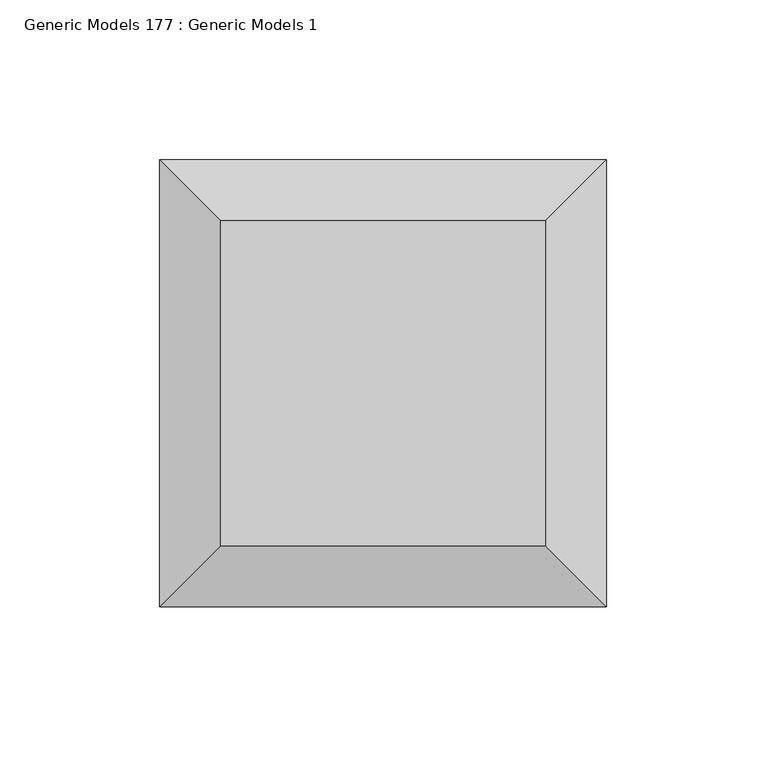
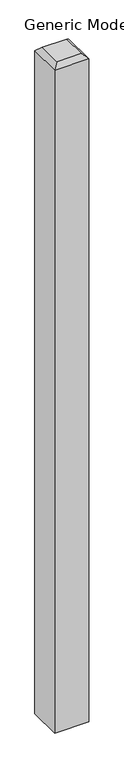
"""IFC4 building model written with IfcOpenShell, lengths in millimetres: proxy geometry, Generic Models 177 : Generic Models 1."""

import ifcopenshell
import ifcopenshell.guid

model = None  # the IFC model being written
_history = None  # IfcOwnerHistory: only IFC2X3 demands one
_inside = {}  # id of a spatial element -> (the spatial element, [elements in it])
_under = {}  # id of a project, library or spatial element -> (it, [spatial elements below it])
_declared = {}  # id of a project -> (the project, [libraries it declares])
_typed = {}  # id of a type object -> (the type object, [elements of that type])
_made_of = {}  # id of a material, layer set ... -> (it, [elements and type objects made of it])


def new_model(schema):
    """Start an empty IFC model of exactly this schema.

    Asked for "IFC4X3", IfcOpenShell would pick the latest addendum, in which some entities
    have other attributes; the version numbers below select the first issue.
    IFC2X3 requires an IfcOwnerHistory on every rooted entity: one is made here for all.
    """
    global model, _history
    if schema == "IFC4X3":
        model = ifcopenshell.file(schema_version=(4, 3, 0, 0))
    else:
        model = ifcopenshell.file(schema=schema)
    _inside.clear()
    _under.clear()
    _declared.clear()
    _typed.clear()
    _made_of.clear()
    _history = None
    if model.schema == "IFC2X3":
        org = make("IfcOrganization", Name="unknown")
        user = make(
            "IfcPersonAndOrganization",
            ThePerson=make("IfcPerson", FamilyName="unknown"),
            TheOrganization=org,
        )
        app = make(
            "IfcApplication",
            ApplicationDeveloper=org,
            Version="unknown",
            ApplicationFullName="unknown",
            ApplicationIdentifier="unknown",
        )
        _history = make(
            "IfcOwnerHistory",
            OwningUser=user,
            OwningApplication=app,
            ChangeAction="ADDED",
            CreationDate=0,
        )
    return model


def make(cls, **values):
    """One entity of the class cls with the attributes given. An attribute that is None is left unset."""
    return model.create_entity(
        cls, **{name: value for name, value in values.items() if value is not None}
    )


def rooted(cls, **values):
    """An entity with a GlobalId (a new one), such as an element, a storey or a relation."""
    return make(cls, GlobalId=ifcopenshell.guid.new(), OwnerHistory=_history, **values)


def si_unit(unit_type, name, prefix=None):
    """IfcSIUnit, for example si_unit("LENGTHUNIT", "METRE", prefix="MILLI")."""
    return make("IfcSIUnit", UnitType=unit_type, Prefix=prefix, Name=name)


def assignment(units):
    """IfcUnitAssignment: the units of a project."""
    return None if units is None else make("IfcUnitAssignment", Units=units)


def point(xyz):
    """IfcCartesianPoint."""
    return None if xyz is None else make("IfcCartesianPoint", Coordinates=xyz)


def direction(xyz):
    """IfcDirection."""
    return None if xyz is None else make("IfcDirection", DirectionRatios=xyz)


def frame(location, z_axis=None, x_axis=None):
    """IfcAxis2Placement3D, a coordinate frame: its origin and axes. An axis left out is left unset."""
    return make(
        "IfcAxis2Placement3D",
        Location=point(location),
        Axis=direction(z_axis),
        RefDirection=direction(x_axis),
    )


def origin():
    """The frame at (0, 0, 0) with its axes left unset."""
    return frame((0.0, 0.0, 0.0))


def place(relative_to, where):
    """IfcLocalPlacement: puts the frame where relative to a parent placement (None: the world)."""
    return make(
        "IfcLocalPlacement", PlacementRelTo=relative_to, RelativePlacement=where
    )


def context(
    kind, dimensions, precision=None, world=None, true_north=None, identifier=None
):
    """IfcGeometricRepresentationContext, for example the 3D "Model" context."""
    return make(
        "IfcGeometricRepresentationContext",
        ContextIdentifier=identifier,
        ContextType=kind,
        CoordinateSpaceDimension=dimensions,
        Precision=precision,
        WorldCoordinateSystem=world,
        TrueNorth=true_north,
    )


def project(units=None, contexts=None):
    """IfcProject with its units and contexts."""
    return rooted(
        "IfcProject",
        Name="project",
        RepresentationContexts=contexts,
        UnitsInContext=assignment(units),
    )


def spatial(cls, under=None, at=None, **own):
    """A site, building, storey or space (cls), placed at a placement, below another one or the project."""
    s = rooted(cls, ObjectPlacement=at, **own)
    if under is not None:
        _under.setdefault(under.id(), (under, []))[1].append(s)
    return s


def faces_of(points, faces, orient=None, outer=None):
    """IfcFace entities. A face is a list of loops; a loop is a list of indices into points, from 0.

    orient and outer hold one flag for each loop. By default every Orientation is true, the
    first loop of a face is its IfcFaceOuterBound and the others are IfcFaceBound.
    """
    made = []
    for i, loops in enumerate(faces):
        bounds = []
        for j, loop in enumerate(loops):
            is_outer = j == 0 if outer is None else outer[i][j]
            bounds.append(
                make(
                    "IfcFaceOuterBound" if is_outer else "IfcFaceBound",
                    Bound=make("IfcPolyLoop", Polygon=[points[k] for k in loop]),
                    Orientation=True if orient is None else orient[i][j],
                )
            )
        made.append(make("IfcFace", Bounds=bounds))
    return made


def faceted_brep(points, faces, orient=None, outer=None, voids=None):
    """IfcFacetedBrep: a solid bounded by flat faces; with voids (closed shells), ...WithVoids."""
    shared = [point(p) for p in points]
    hull = make("IfcClosedShell", CfsFaces=faces_of(shared, faces, orient, outer))
    if voids is None:
        return make("IfcFacetedBrep", Outer=hull)
    return make(
        "IfcFacetedBrepWithVoids",
        Outer=hull,
        Voids=[
            make(cls, CfsFaces=faces_of(shared, fs, o, b)) for cls, fs, o, b in voids
        ],
    )


def shape(context_of_items, identifier, shape_type, items):
    """IfcShapeRepresentation: the items that make up one representation, for example the "Body"."""
    return make(
        "IfcShapeRepresentation",
        ContextOfItems=context_of_items,
        RepresentationIdentifier=identifier,
        RepresentationType=shape_type,
        Items=items,
    )


def source(mapping_origin, context_of_items, identifier, shape_type, items):
    """IfcRepresentationMap: a shape defined once, which mapped items show again and again."""
    return make(
        "IfcRepresentationMap",
        MappingOrigin=mapping_origin,
        MappedRepresentation=shape(context_of_items, identifier, shape_type, items),
    )


def transform(
    local_origin,
    x_axis=None,
    y_axis=None,
    z_axis=None,
    scale=None,
    scale2=None,
    scale3=None,
    uniform=True,
):
    """IfcCartesianTransformationOperator3D, or its non-uniform kind. x_axis, y_axis, z_axis: its Axis1, 2, 3."""
    if uniform:
        return make(
            "IfcCartesianTransformationOperator3D",
            Axis1=direction(x_axis),
            Axis2=direction(y_axis),
            LocalOrigin=point(local_origin),
            Scale=scale,
            Axis3=direction(z_axis),
        )
    return make(
        "IfcCartesianTransformationOperator3DnonUniform",
        Axis1=direction(x_axis),
        Axis2=direction(y_axis),
        LocalOrigin=point(local_origin),
        Scale=scale,
        Axis3=direction(z_axis),
        Scale2=scale2,
        Scale3=scale3,
    )


def mapped(mapping_source, mapping_target):
    """IfcMappedItem: shows the shape of a source again, moved by a transform."""
    return make(
        "IfcMappedItem", MappingSource=mapping_source, MappingTarget=mapping_target
    )


def made_of(thing, what):
    """Note that an element or type object is made of a material, layer set ...; save() writes the relation."""
    if what is not None:
        _made_of.setdefault(what.id(), (what, []))[1].append(thing)
    return thing


def element(
    cls,
    number,
    at=None,
    inside=None,
    cuts=None,
    type_object=None,
    material=None,
    context=None,
    identifier="Body",
    shape_type=None,
    held_by="IfcProductDefinitionShape",
    body=None,
    shapes=None,
    **own,
):
    """One element of the class cls, such as IfcWall. Its Tag is "e" and its number.

    at: its placement. inside: the storey or other place that contains it. cuts: it is an
    opening in that element (IfcRelVoidsElement). A single representation is given by context,
    identifier, shape_type and body (its items); several are given by shapes. held_by: the class
    of the entity that holds the representations. save() writes the other relations.
    """
    e = rooted(cls, Tag="e%d" % number, ObjectPlacement=at, **own)
    if body is not None:
        shapes = [shape(context, identifier, shape_type, body)]
    if shapes is not None:
        e.Representation = make(held_by, Representations=shapes)
    if inside is not None:
        _inside.setdefault(inside.id(), (inside, []))[1].append(e)
    if cuts is not None:
        rooted(
            "IfcRelVoidsElement", RelatingBuildingElement=cuts, RelatedOpeningElement=e
        )
    if type_object is not None:
        _typed.setdefault(type_object.id(), (type_object, []))[1].append(e)
    return made_of(e, material)


def aggregate(whole, parts):
    """IfcRelAggregates: a whole, such as a stair, and the parts it consists of."""
    return rooted("IfcRelAggregates", RelatingObject=whole, RelatedObjects=parts)


def save(model, path):
    """Write the relations noted so far, then the file.

    IfcRelAggregates (storeys below a building ...), IfcRelContainedInSpatialStructure (elements
    in a storey), IfcRelDefinesByType, IfcRelAssociatesMaterial and IfcRelDeclares: one each for
    every whole, place, type object, material and project.
    """
    for whole, parts in _under.values():
        aggregate(whole, parts)
    for where, things in _inside.values():
        rooted(
            "IfcRelContainedInSpatialStructure",
            RelatedElements=things,
            RelatingStructure=where,
        )
    for kind, things in _typed.values():
        rooted("IfcRelDefinesByType", RelatedObjects=things, RelatingType=kind)
    for what, things in _made_of.values():
        rooted("IfcRelAssociatesMaterial", RelatedObjects=things, RelatingMaterial=what)
    for by, libraries in _declared.values():
        rooted("IfcRelDeclares", RelatingContext=by, RelatedDefinitions=libraries)
    model.write(path)


def generic_models_177_generic_models_1_1d143019(model_context):
    return source(origin(), model_context, "Body", "Brep", [
        faceted_brep([(56665.8125, 528.6375, -1066.8), (56526.1125, 528.6375, -1066.8), (56526.1125, 528.6375, 1809.75), (56665.8125, 528.6375, 1809.75), (56665.8125, 388.9375, -1066.8), (56665.8125, 388.9375, 1809.75), (56526.1125, 388.9375, 1809.75), (56526.1125, 388.9375, -1066.8), (56545.1625, 407.9875, 1828.8), (56646.7625, 407.9875, 1828.8), (56646.7625, 509.5875, 1828.8), (56545.1625, 509.5875, 1828.8)], [[[0, 1, 2, 3]], [[4, 5, 6, 7]], [[1, 0, 4, 7]], [[2, 1, 7, 6]], [[8, 9, 10, 11]], [[0, 3, 5, 4]], [[2, 6, 8, 11]], [[5, 3, 10, 9]], [[6, 5, 9, 8]], [[3, 2, 11, 10]]]),
    ])


if __name__ == "__main__":
    model = new_model("IFC4")
    model_context = context("Model", 3, world=origin())
    ifc_project = project(units=[si_unit("LENGTHUNIT", "METRE", prefix="MILLI")], contexts=[model_context])
    site = spatial("IfcSite", under=ifc_project)
    building = spatial("IfcBuilding", under=site)
    placement = place(None, origin())
    generic_models_177_generic_models_1_shape = generic_models_177_generic_models_1_1d143019(model_context)
    element("IfcBuildingElementProxy", 1, Name="Generic Models 177 : Generic Models 1", ObjectType="Generic Models 177 : Generic Models 1", at=placement, inside=building, context=model_context, shape_type="MappedRepresentation", body=[
        mapped(generic_models_177_generic_models_1_shape, transform((0.0, 0.0, 0.0), x_axis=(1.0, 0.0, 0.0), y_axis=(0.0, 1.0, 0.0), z_axis=(0.0, 0.0, 1.0))),
    ])
    save(model, "model.ifc")

# Revit data of these elements
# Element 1 (IfcBuildingElementProxy, "Generic Models 177 : Generic Models 1")
#   Materials on its faces: "TREATED CEDAR 6X6 POST"
# Materials
#   "TREATED CEDAR 6X6 POST": class "Wood", colour RGB 234 198 147, transparency 0, Description = "Pinus Echinata", Cost = 0
